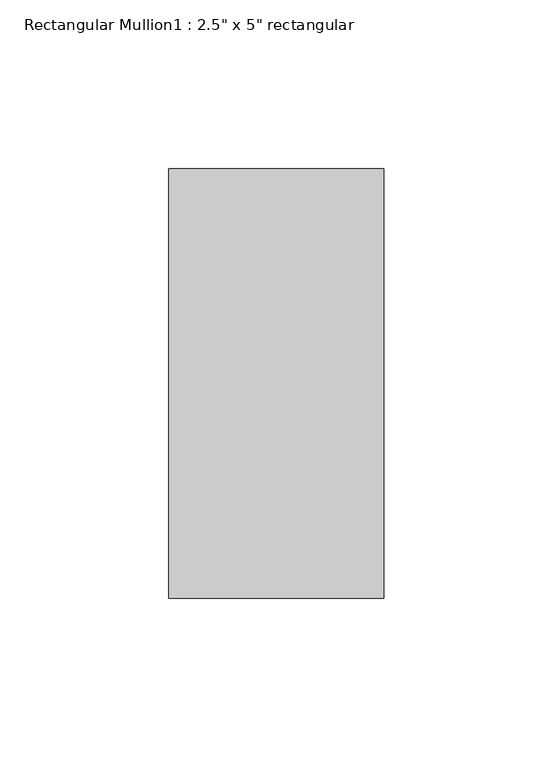
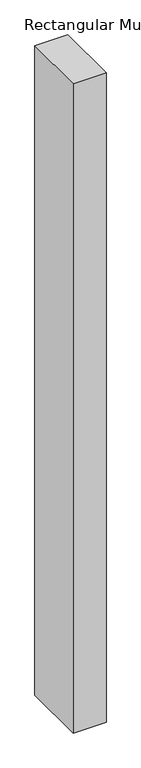
"""IFC4 building model written with IfcOpenShell, lengths in millimetres: member geometry."""

from ifc_helpers import new_model, si_unit, frame, origin, place, context, project, spatial, polyline, outline, extrude, source, transform, mapped, element, save


def member_c609194f(model_context):
    return source(origin(), model_context, "Body", "SweptSolid", [
        extrude(outline(polyline([(31.75, 63.5), (31.75, -63.5), (-31.75, -63.5), (-31.75, 63.5), (31.75, 63.5)])), frame((0.0, 0.0, -1320.067308), z_axis=(0.0, 0.0, 1.0), x_axis=(1.0, 0.0, 0.0)), (0.0, 0.0, 1.0), 1320.067308),
    ])


if __name__ == "__main__":
    model = new_model("IFC4")
    model_context = context("Model", 3, world=origin())
    ifc_project = project(units=[si_unit("LENGTHUNIT", "METRE", prefix="MILLI")], contexts=[model_context])
    site = spatial("IfcSite", under=ifc_project)
    building = spatial("IfcBuilding", under=site)
    placement = place(None, origin())
    member_shape = member_c609194f(model_context)
    element("IfcMember", 1, ObjectType="Rectangular Mullion1 : 2.5\" x 5\" rectangular", at=placement, inside=building, context=model_context, shape_type="MappedRepresentation", body=[
        mapped(member_shape, transform((0.0, 0.0, 0.0), x_axis=(1.0, 0.0, 0.0), y_axis=(0.0, 1.0, 0.0), z_axis=(0.0, 0.0, 1.0))),
    ])
    save(model, "model.ifc")

# Revit data of these elements
# Type "Rectangular Mullion1 : 2.5\" x 5\" rectangular"
#   built-in parameter 1007304 = 0.416667 (stored number, unit not read)
#   built-in parameter 1007301 = 0.104167 (stored number, unit not read)
#   built-in parameter 1007300 = 0.104167 (stored number, unit not read)
# Element 1 (IfcMember, "Rectangular Mullion1 : 2.5\" x 5\" rectangular")
#   Materials on its faces: "support-frame"
# Materials
#   "support-frame": class "Unassigned", colour RGB 233 233 233, transparency 0, Cost = 0
